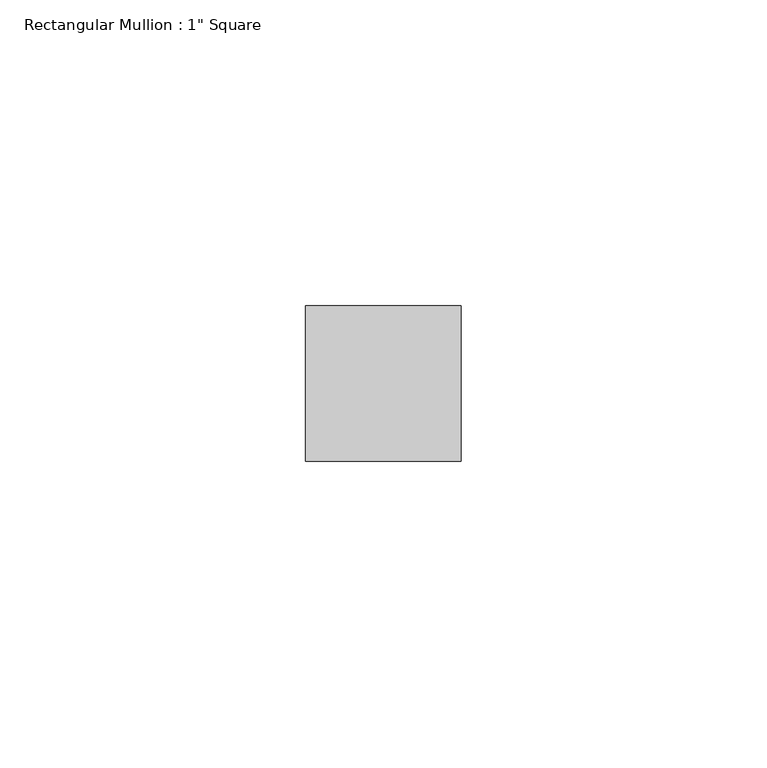
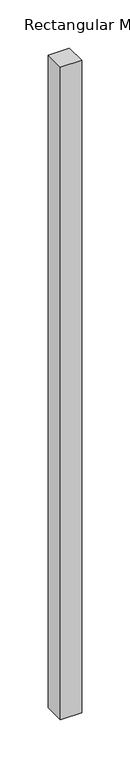
"""IFC4 building model written with IfcOpenShell, lengths in millimetres: member geometry."""

from ifc_helpers import new_model, si_unit, frame, origin, place, context, project, spatial, polyline, outline, extrude, source, transform, mapped, element, save


def member_3fb67473(model_context):
    return source(origin(), model_context, "Body", "SweptSolid", [
        extrude(outline(polyline([(0.0, 12.7), (0.0, -12.7), (-25.4, -12.7), (-25.4, 12.7), (0.0, 12.7)])), frame((0.0, 0.0, -825.5), z_axis=(0.0, 0.0, 1.0), x_axis=(1.0, 0.0, 0.0)), (0.0, 0.0, 1.0), 825.5),
    ])


if __name__ == "__main__":
    model = new_model("IFC4")
    model_context = context("Model", 3, world=origin())
    ifc_project = project(units=[si_unit("LENGTHUNIT", "METRE", prefix="MILLI")], contexts=[model_context])
    site = spatial("IfcSite", under=ifc_project)
    building = spatial("IfcBuilding", under=site)
    placement = place(None, origin())
    member_shape = member_3fb67473(model_context)
    element("IfcMember", 1, ObjectType="Rectangular Mullion : 1\" Square", at=placement, inside=building, context=model_context, shape_type="MappedRepresentation", body=[
        mapped(member_shape, transform((0.0, 0.0, 0.0), x_axis=(1.0, 0.0, 0.0), y_axis=(0.0, 1.0, 0.0), z_axis=(0.0, 0.0, 1.0))),
    ])
    save(model, "model.ifc")

# Revit data of these elements
# Type "Rectangular Mullion : 1\" Square"
#   built-in parameter 1007304 = 0.0833333 (stored number, unit not read)
#   built-in parameter 1007301 = 0.0416667 (stored number, unit not read)
#   built-in parameter 1007300 = 0.0416667 (stored number, unit not read)
# Element 1 (IfcMember, "Rectangular Mullion : 1\" Square")
#   Materials on its faces: "Metal - Aluminum"
# Materials
#   "Metal - Aluminum": class "Metal", colour RGB 247 247 247, transparency 0
